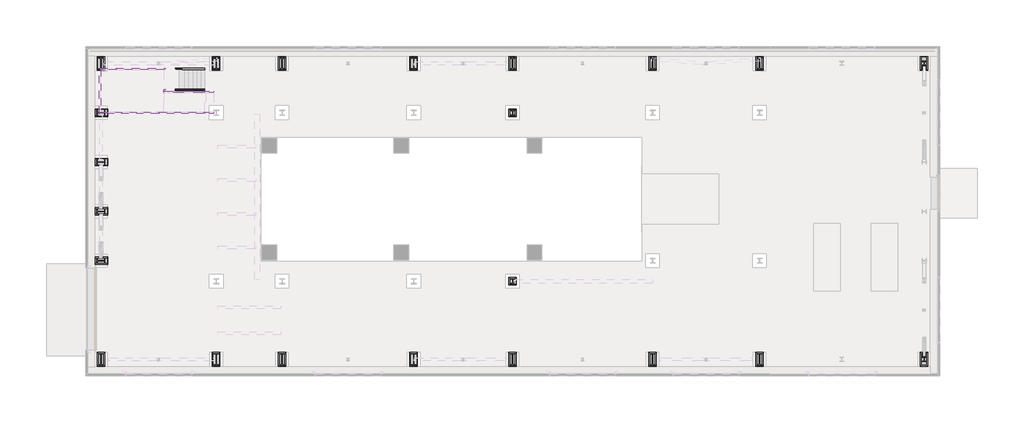
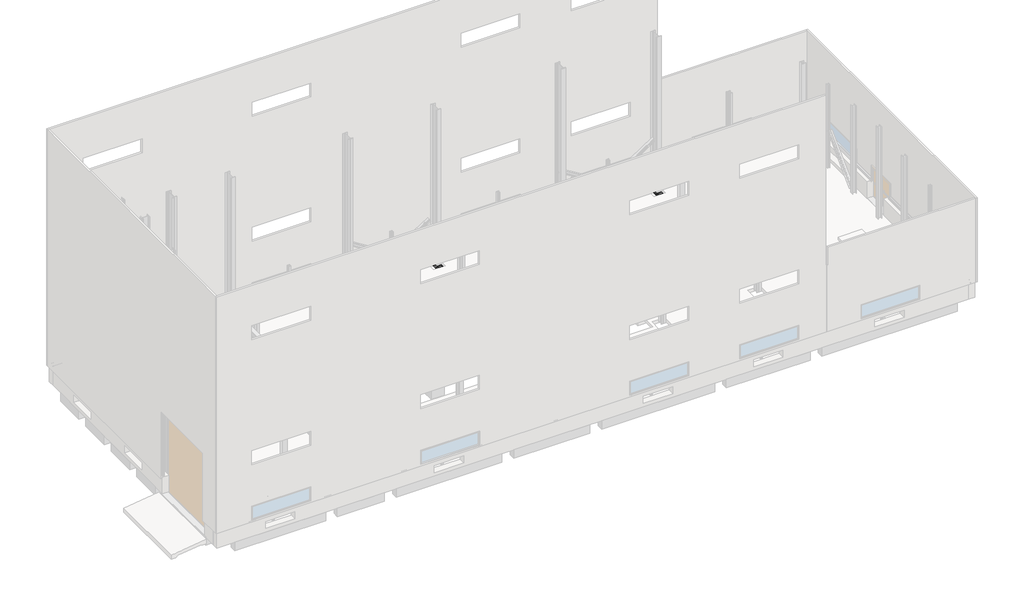
# One storey, part 4 of 4: 23 proxies, 10 members.
# Revit data of these elements (continued)
# Type "그라우트9 : 그라우트"
#   Description = ""
# Type "C-250X90"
#   Keynote = "ㄷ-250×90x9x13"
# Element 1 (IfcBuildingElementProxy, "그라우트 : 그라우트")
#   Phase Created = New Construction
# Element 2 (IfcBuildingElementProxy, "그라우트2 : 그라우트")
#   Phase Created = New Construction
# Element 3 (IfcBuildingElementProxy, "그라우트3 : 그라우트")
#   Phase Created = New Construction
# Element 4 (IfcBuildingElementProxy, "그라우트4 : 그라우트")
#   Phase Created = New Construction
# Element 5 (IfcBuildingElementProxy, "그라우트5 : 그라우트")
#   Phase Created = New Construction
# Element 6 (IfcBuildingElementProxy, "그라우트6 : 그라우트")
#   Phase Created = New Construction
# Element 7 (IfcBuildingElementProxy, "그라우트7 : 그라우트")
#   Phase Created = New Construction
# Element 8 (IfcBuildingElementProxy, "그라우트8 : 그라우트")
#   Phase Created = New Construction
# Element 9 (IfcBuildingElementProxy, "그라우트9 : 그라우트")
#   Phase Created = New Construction
# Element 10 (IfcBuildingElementProxy, "그라우트10 : 그라우트")
#   Phase Created = New Construction
# Element 11 (IfcBuildingElementProxy, "그라우트11 : 그라우트")
#   Phase Created = New Construction
# Element 12 (IfcBuildingElementProxy, "그라우트12 : 그라우트")
#   Phase Created = New Construction
# Element 13 (IfcBuildingElementProxy, "그라우트13 : 그라우트")
#   Phase Created = New Construction
# Element 14 (IfcBuildingElementProxy, "그라우트14 : 그라우트")
#   Phase Created = New Construction
# Element 15 (IfcBuildingElementProxy, "그라우트15 : 그라우트")
#   Phase Created = New Construction
# Element 16 (IfcBuildingElementProxy, "그라우트16 : 그라우트")
#   Phase Created = New Construction
# Element 17 (IfcBuildingElementProxy, "그라우트17 : 그라우트")
#   Phase Created = New Construction
# Element 18 (IfcBuildingElementProxy, "그라우트18 : 그라우트")
#   Phase Created = New Construction
# Element 19 (IfcBuildingElementProxy, "그라우트20 : 그라우트")
#   Phase Created = New Construction
# Element 20 (IfcBuildingElementProxy, "그라우트22 : 그라우트")
#   Phase Created = New Construction
# Element 21 (IfcBuildingElementProxy, "그라우트23 : 그라우트")
#   Phase Created = New Construction
# Element 22 (IfcBuildingElementProxy, "그라우트19 : 그라우트")
#   Phase Created = New Construction
# Element 23 (IfcBuildingElementProxy, "Grout : H_GM_AMM_Grouting_T50")
#   Phase Created = New Construction
# Elements 24, 25, 26, 27, 28, 29, 30, 31, 32, 33 (IfcMember, "C-250X90")
#   Mark = "ST1"
#   Phase Created = New Construction
#   Materials on its faces: "SM490"
# Materials
#   "SM490": class "Unassigned", colour RGB 84 83 81, transparency 0
# Room at (31078.827, 30248.358) mm, phase "New Construction", upper level "1ST T.O.C", upper offset 2.0000 m, lower offset 0.0000 m
#   Comments = ""
#   Number = "101"
#   Name = "TURBINE HALL"
